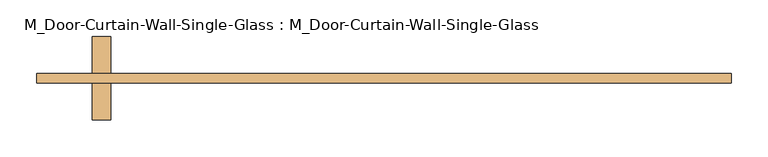
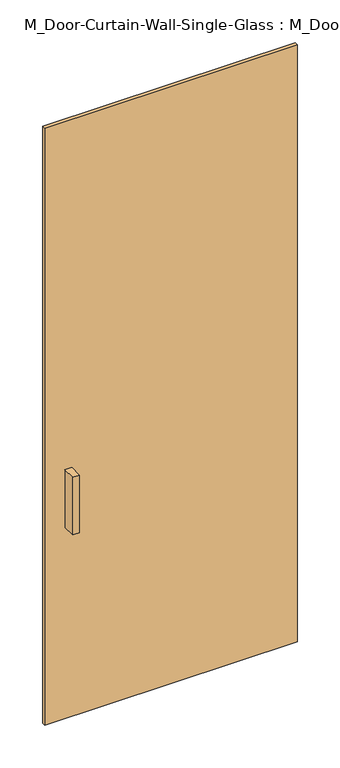
"""IFC4 building model written with IfcOpenShell, lengths in millimetres: door geometry, M_Door-Curtain-Wall-Single-Glass : M_Door-Curtain-Wall-Single-Glass."""

import ifcopenshell
import ifcopenshell.guid

model = None  # the IFC model being written
_history = None  # IfcOwnerHistory: only IFC2X3 demands one
_inside = {}  # id of a spatial element -> (the spatial element, [elements in it])
_under = {}  # id of a project, library or spatial element -> (it, [spatial elements below it])
_declared = {}  # id of a project -> (the project, [libraries it declares])
_typed = {}  # id of a type object -> (the type object, [elements of that type])
_made_of = {}  # id of a material, layer set ... -> (it, [elements and type objects made of it])


def new_model(schema):
    """Start an empty IFC model of exactly this schema.

    Asked for "IFC4X3", IfcOpenShell would pick the latest addendum, in which some entities
    have other attributes; the version numbers below select the first issue.
    IFC2X3 requires an IfcOwnerHistory on every rooted entity: one is made here for all.
    """
    global model, _history
    if schema == "IFC4X3":
        model = ifcopenshell.file(schema_version=(4, 3, 0, 0))
    else:
        model = ifcopenshell.file(schema=schema)
    _inside.clear()
    _under.clear()
    _declared.clear()
    _typed.clear()
    _made_of.clear()
    _history = None
    if model.schema == "IFC2X3":
        org = make("IfcOrganization", Name="unknown")
        user = make(
            "IfcPersonAndOrganization",
            ThePerson=make("IfcPerson", FamilyName="unknown"),
            TheOrganization=org,
        )
        app = make(
            "IfcApplication",
            ApplicationDeveloper=org,
            Version="unknown",
            ApplicationFullName="unknown",
            ApplicationIdentifier="unknown",
        )
        _history = make(
            "IfcOwnerHistory",
            OwningUser=user,
            OwningApplication=app,
            ChangeAction="ADDED",
            CreationDate=0,
        )
    return model


def make(cls, **values):
    """One entity of the class cls with the attributes given. An attribute that is None is left unset."""
    return model.create_entity(
        cls, **{name: value for name, value in values.items() if value is not None}
    )


def rooted(cls, **values):
    """An entity with a GlobalId (a new one), such as an element, a storey or a relation."""
    return make(cls, GlobalId=ifcopenshell.guid.new(), OwnerHistory=_history, **values)


def si_unit(unit_type, name, prefix=None):
    """IfcSIUnit, for example si_unit("LENGTHUNIT", "METRE", prefix="MILLI")."""
    return make("IfcSIUnit", UnitType=unit_type, Prefix=prefix, Name=name)


def assignment(units):
    """IfcUnitAssignment: the units of a project."""
    return None if units is None else make("IfcUnitAssignment", Units=units)


def point(xyz):
    """IfcCartesianPoint."""
    return None if xyz is None else make("IfcCartesianPoint", Coordinates=xyz)


def direction(xyz):
    """IfcDirection."""
    return None if xyz is None else make("IfcDirection", DirectionRatios=xyz)


def frame(location, z_axis=None, x_axis=None):
    """IfcAxis2Placement3D, a coordinate frame: its origin and axes. An axis left out is left unset."""
    return make(
        "IfcAxis2Placement3D",
        Location=point(location),
        Axis=direction(z_axis),
        RefDirection=direction(x_axis),
    )


def origin():
    """The frame at (0, 0, 0) with its axes left unset."""
    return frame((0.0, 0.0, 0.0))


def origin_with_axes():
    """The frame at (0, 0, 0) with the z axis (0, 0, 1) and the x axis (1, 0, 0) written out."""
    return frame((0.0, 0.0, 0.0), z_axis=(0.0, 0.0, 1.0), x_axis=(1.0, 0.0, 0.0))


def place(relative_to, where):
    """IfcLocalPlacement: puts the frame where relative to a parent placement (None: the world)."""
    return make(
        "IfcLocalPlacement", PlacementRelTo=relative_to, RelativePlacement=where
    )


def context(
    kind, dimensions, precision=None, world=None, true_north=None, identifier=None
):
    """IfcGeometricRepresentationContext, for example the 3D "Model" context."""
    return make(
        "IfcGeometricRepresentationContext",
        ContextIdentifier=identifier,
        ContextType=kind,
        CoordinateSpaceDimension=dimensions,
        Precision=precision,
        WorldCoordinateSystem=world,
        TrueNorth=true_north,
    )


def project(units=None, contexts=None):
    """IfcProject with its units and contexts."""
    return rooted(
        "IfcProject",
        Name="project",
        RepresentationContexts=contexts,
        UnitsInContext=assignment(units),
    )


def spatial(cls, under=None, at=None, **own):
    """A site, building, storey or space (cls), placed at a placement, below another one or the project."""
    s = rooted(cls, ObjectPlacement=at, **own)
    if under is not None:
        _under.setdefault(under.id(), (under, []))[1].append(s)
    return s


def polyline(points):
    """IfcPolyline through the points."""
    return make("IfcPolyline", Points=[point(p) for p in points])


def outline(outer, holes=None, kind="AREA"):
    """IfcArbitraryClosedProfileDef: a profile drawn as a closed curve; with holes, ...WithVoids."""
    if holes is None:
        return make("IfcArbitraryClosedProfileDef", ProfileType=kind, OuterCurve=outer)
    return make(
        "IfcArbitraryProfileDefWithVoids",
        ProfileType=kind,
        OuterCurve=outer,
        InnerCurves=holes,
    )


def extrude(swept, where, along, depth):
    """IfcExtrudedAreaSolid: the profile swept, set in the frame where, extruded along a direction by depth."""
    return make(
        "IfcExtrudedAreaSolid",
        SweptArea=swept,
        Position=where,
        ExtrudedDirection=direction(along),
        Depth=depth,
    )


def shape(context_of_items, identifier, shape_type, items):
    """IfcShapeRepresentation: the items that make up one representation, for example the "Body"."""
    return make(
        "IfcShapeRepresentation",
        ContextOfItems=context_of_items,
        RepresentationIdentifier=identifier,
        RepresentationType=shape_type,
        Items=items,
    )


def source(mapping_origin, context_of_items, identifier, shape_type, items):
    """IfcRepresentationMap: a shape defined once, which mapped items show again and again."""
    return make(
        "IfcRepresentationMap",
        MappingOrigin=mapping_origin,
        MappedRepresentation=shape(context_of_items, identifier, shape_type, items),
    )


def transform(
    local_origin,
    x_axis=None,
    y_axis=None,
    z_axis=None,
    scale=None,
    scale2=None,
    scale3=None,
    uniform=True,
):
    """IfcCartesianTransformationOperator3D, or its non-uniform kind. x_axis, y_axis, z_axis: its Axis1, 2, 3."""
    if uniform:
        return make(
            "IfcCartesianTransformationOperator3D",
            Axis1=direction(x_axis),
            Axis2=direction(y_axis),
            LocalOrigin=point(local_origin),
            Scale=scale,
            Axis3=direction(z_axis),
        )
    return make(
        "IfcCartesianTransformationOperator3DnonUniform",
        Axis1=direction(x_axis),
        Axis2=direction(y_axis),
        LocalOrigin=point(local_origin),
        Scale=scale,
        Axis3=direction(z_axis),
        Scale2=scale2,
        Scale3=scale3,
    )


def mapped(mapping_source, mapping_target):
    """IfcMappedItem: shows the shape of a source again, moved by a transform."""
    return make(
        "IfcMappedItem", MappingSource=mapping_source, MappingTarget=mapping_target
    )


def made_of(thing, what):
    """Note that an element or type object is made of a material, layer set ...; save() writes the relation."""
    if what is not None:
        _made_of.setdefault(what.id(), (what, []))[1].append(thing)
    return thing


def element(
    cls,
    number,
    at=None,
    inside=None,
    cuts=None,
    type_object=None,
    material=None,
    context=None,
    identifier="Body",
    shape_type=None,
    held_by="IfcProductDefinitionShape",
    body=None,
    shapes=None,
    **own,
):
    """One element of the class cls, such as IfcWall. Its Tag is "e" and its number.

    at: its placement. inside: the storey or other place that contains it. cuts: it is an
    opening in that element (IfcRelVoidsElement). A single representation is given by context,
    identifier, shape_type and body (its items); several are given by shapes. held_by: the class
    of the entity that holds the representations. save() writes the other relations.
    """
    e = rooted(cls, Tag="e%d" % number, ObjectPlacement=at, **own)
    if body is not None:
        shapes = [shape(context, identifier, shape_type, body)]
    if shapes is not None:
        e.Representation = make(held_by, Representations=shapes)
    if inside is not None:
        _inside.setdefault(inside.id(), (inside, []))[1].append(e)
    if cuts is not None:
        rooted(
            "IfcRelVoidsElement", RelatingBuildingElement=cuts, RelatedOpeningElement=e
        )
    if type_object is not None:
        _typed.setdefault(type_object.id(), (type_object, []))[1].append(e)
    return made_of(e, material)


def aggregate(whole, parts):
    """IfcRelAggregates: a whole, such as a stair, and the parts it consists of."""
    return rooted("IfcRelAggregates", RelatingObject=whole, RelatedObjects=parts)


def save(model, path):
    """Write the relations noted so far, then the file.

    IfcRelAggregates (storeys below a building ...), IfcRelContainedInSpatialStructure (elements
    in a storey), IfcRelDefinesByType, IfcRelAssociatesMaterial and IfcRelDeclares: one each for
    every whole, place, type object, material and project.
    """
    for whole, parts in _under.values():
        aggregate(whole, parts)
    for where, things in _inside.values():
        rooted(
            "IfcRelContainedInSpatialStructure",
            RelatedElements=things,
            RelatingStructure=where,
        )
    for kind, things in _typed.values():
        rooted("IfcRelDefinesByType", RelatedObjects=things, RelatingType=kind)
    for what, things in _made_of.values():
        rooted("IfcRelAssociatesMaterial", RelatedObjects=things, RelatingMaterial=what)
    for by, libraries in _declared.values():
        rooted("IfcRelDeclares", RelatingContext=by, RelatedDefinitions=libraries)
    model.write(path)


def m_door_curtain_wall_single_glass_m_door_curtain_wall_single_3c5a18a5(model_context):
    return source(origin(), model_context, "Body", "SweptSolid", [
        extrude(outline(polyline([(475.0, 50.8), (475.0, 38.1), (-475.0, 38.1), (-475.0, 50.8), (475.0, 50.8)])), origin_with_axes(), (0.0, 0.0, 1.0), 2375.0),
        extrude(outline(polyline([(-373.4, -12.7), (-398.8, -12.7), (-398.8, 38.1), (-373.4, 38.1), (-373.4, -12.7)])), frame((0.0, 0.0, 762.0), z_axis=(0.0, 0.0, 1.0), x_axis=(1.0, 0.0, 0.0)), (0.0, 0.0, 1.0), 228.6),
        extrude(outline(polyline([(-398.8, 101.6), (-373.4, 101.6), (-373.4, 50.8), (-398.8, 50.8), (-398.8, 101.6)])), frame((0.0, 0.0, 762.0), z_axis=(0.0, 0.0, 1.0), x_axis=(1.0, 0.0, 0.0)), (0.0, 0.0, 1.0), 228.6),
    ])


if __name__ == "__main__":
    model = new_model("IFC4")
    model_context = context("Model", 3, world=origin())
    ifc_project = project(units=[si_unit("LENGTHUNIT", "METRE", prefix="MILLI")], contexts=[model_context])
    site = spatial("IfcSite", under=ifc_project)
    building = spatial("IfcBuilding", under=site)
    placement = place(None, origin())
    m_door_curtain_wall_single_glass_m_door_curtain_wall_single_shape = m_door_curtain_wall_single_glass_m_door_curtain_wall_single_3c5a18a5(model_context)
    element("IfcDoor", 1, ObjectType="M_Door-Curtain-Wall-Single-Glass : M_Door-Curtain-Wall-Single-Glass", at=placement, inside=building, context=model_context, shape_type="MappedRepresentation", body=[
        mapped(m_door_curtain_wall_single_glass_m_door_curtain_wall_single_shape, transform((0.0, 0.0, 0.0), x_axis=(1.0, 0.0, 0.0), y_axis=(0.0, 1.0, 0.0), z_axis=(0.0, 0.0, 1.0))),
    ])
    save(model, "model.ifc")

# Revit data of these elements
# Type "M_Door-Curtain-Wall-Single-Glass : M_Door-Curtain-Wall-Single-Glass"
#   Type Mark = "50"
#   Assembly Code = "B2030100"
#   Analytic Construction = "<None>"
#   Width [instance default] = 900 mm
#   Thermal Resistance (R) = 1.7611 (m²·K)/W
#   Swing Angle [instance default] = 90.00°
#   Heat Transfer Coefficient (U) = 0.567826 W/(m²·K)
#   Offset = 50.8 mm
#   Define Thermal Properties by = 1
#   Function = 1
#   Door Handle Material = Aluminum
#   Glazing = Glass
#   Visual Light Transmittance = 0
#   Solar Heat Gain Coefficient = 0
#   Construction Type Id = ""
# Element 1 (IfcDoor, "M_Door-Curtain-Wall-Single-Glass : M_Door-Curtain-Wall-Single-Glass")
#   Width = 950 mm
#   Materials on its faces: "Aluminum", "Glass"
# Materials
#   "Aluminum": class "Metal", colour RGB 247 247 247, transparency 0, Description = "Aluminum 6061", Cost = 0
#   "Glass": class "Glass", colour RGB 0 128 192, transparency 0.9, Description = "Soda Lime Glass", Cost = 0
